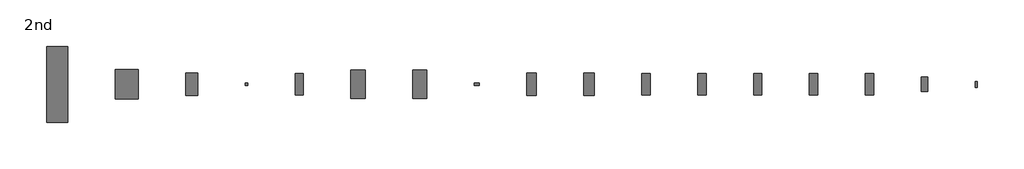
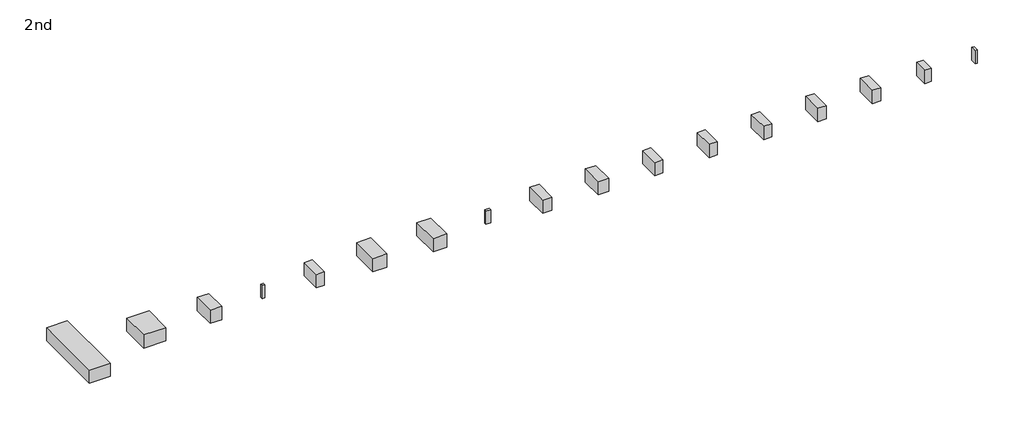
# One storey: 17 proxies.
"""IFC4 building model written with IfcOpenShell, lengths in millimetres."""

import ifcopenshell
import ifcopenshell.guid

model = None  # the IFC model being written
_history = None  # IfcOwnerHistory: only IFC2X3 demands one
_inside = {}  # id of a spatial element -> (the spatial element, [elements in it])
_under = {}  # id of a project, library or spatial element -> (it, [spatial elements below it])
_declared = {}  # id of a project -> (the project, [libraries it declares])
_typed = {}  # id of a type object -> (the type object, [elements of that type])
_made_of = {}  # id of a material, layer set ... -> (it, [elements and type objects made of it])


def new_model(schema):
    """Start an empty IFC model of exactly this schema.

    Asked for "IFC4X3", IfcOpenShell would pick the latest addendum, in which some entities
    have other attributes; the version numbers below select the first issue.
    IFC2X3 requires an IfcOwnerHistory on every rooted entity: one is made here for all.
    """
    global model, _history
    if schema == "IFC4X3":
        model = ifcopenshell.file(schema_version=(4, 3, 0, 0))
    else:
        model = ifcopenshell.file(schema=schema)
    _inside.clear()
    _under.clear()
    _declared.clear()
    _typed.clear()
    _made_of.clear()
    _history = None
    if model.schema == "IFC2X3":
        org = make("IfcOrganization", Name="unknown")
        user = make(
            "IfcPersonAndOrganization",
            ThePerson=make("IfcPerson", FamilyName="unknown"),
            TheOrganization=org,
        )
        app = make(
            "IfcApplication",
            ApplicationDeveloper=org,
            Version="unknown",
            ApplicationFullName="unknown",
            ApplicationIdentifier="unknown",
        )
        _history = make(
            "IfcOwnerHistory",
            OwningUser=user,
            OwningApplication=app,
            ChangeAction="ADDED",
            CreationDate=0,
        )
    return model


def make(cls, **values):
    """One entity of the class cls with the attributes given. An attribute that is None is left unset."""
    return model.create_entity(
        cls, **{name: value for name, value in values.items() if value is not None}
    )


def rooted(cls, **values):
    """An entity with a GlobalId (a new one), such as an element, a storey or a relation."""
    return make(cls, GlobalId=ifcopenshell.guid.new(), OwnerHistory=_history, **values)


def si_unit(unit_type, name, prefix=None):
    """IfcSIUnit, for example si_unit("LENGTHUNIT", "METRE", prefix="MILLI")."""
    return make("IfcSIUnit", UnitType=unit_type, Prefix=prefix, Name=name)


def assignment(units):
    """IfcUnitAssignment: the units of a project."""
    return None if units is None else make("IfcUnitAssignment", Units=units)


def point(xyz):
    """IfcCartesianPoint."""
    return None if xyz is None else make("IfcCartesianPoint", Coordinates=xyz)


def direction(xyz):
    """IfcDirection."""
    return None if xyz is None else make("IfcDirection", DirectionRatios=xyz)


def frame(location, z_axis=None, x_axis=None):
    """IfcAxis2Placement3D, a coordinate frame: its origin and axes. An axis left out is left unset."""
    return make(
        "IfcAxis2Placement3D",
        Location=point(location),
        Axis=direction(z_axis),
        RefDirection=direction(x_axis),
    )


def origin():
    """The frame at (0, 0, 0) with its axes left unset."""
    return frame((0.0, 0.0, 0.0))


def origin_with_axes():
    """The frame at (0, 0, 0) with the z axis (0, 0, 1) and the x axis (1, 0, 0) written out."""
    return frame((0.0, 0.0, 0.0), z_axis=(0.0, 0.0, 1.0), x_axis=(1.0, 0.0, 0.0))


def place(relative_to, where):
    """IfcLocalPlacement: puts the frame where relative to a parent placement (None: the world)."""
    return make(
        "IfcLocalPlacement", PlacementRelTo=relative_to, RelativePlacement=where
    )


def context(
    kind, dimensions, precision=None, world=None, true_north=None, identifier=None
):
    """IfcGeometricRepresentationContext, for example the 3D "Model" context."""
    return make(
        "IfcGeometricRepresentationContext",
        ContextIdentifier=identifier,
        ContextType=kind,
        CoordinateSpaceDimension=dimensions,
        Precision=precision,
        WorldCoordinateSystem=world,
        TrueNorth=true_north,
    )


def project(units=None, contexts=None):
    """IfcProject with its units and contexts."""
    return rooted(
        "IfcProject",
        Name="project",
        RepresentationContexts=contexts,
        UnitsInContext=assignment(units),
    )


def spatial(cls, under=None, at=None, **own):
    """A site, building, storey or space (cls), placed at a placement, below another one or the project."""
    s = rooted(cls, ObjectPlacement=at, **own)
    if under is not None:
        _under.setdefault(under.id(), (under, []))[1].append(s)
    return s


def polyline(points):
    """IfcPolyline through the points."""
    return make("IfcPolyline", Points=[point(p) for p in points])


def outline(outer, holes=None, kind="AREA"):
    """IfcArbitraryClosedProfileDef: a profile drawn as a closed curve; with holes, ...WithVoids."""
    if holes is None:
        return make("IfcArbitraryClosedProfileDef", ProfileType=kind, OuterCurve=outer)
    return make(
        "IfcArbitraryProfileDefWithVoids",
        ProfileType=kind,
        OuterCurve=outer,
        InnerCurves=holes,
    )


def extrude(swept, where, along, depth):
    """IfcExtrudedAreaSolid: the profile swept, set in the frame where, extruded along a direction by depth."""
    return make(
        "IfcExtrudedAreaSolid",
        SweptArea=swept,
        Position=where,
        ExtrudedDirection=direction(along),
        Depth=depth,
    )


def shape(context_of_items, identifier, shape_type, items):
    """IfcShapeRepresentation: the items that make up one representation, for example the "Body"."""
    return make(
        "IfcShapeRepresentation",
        ContextOfItems=context_of_items,
        RepresentationIdentifier=identifier,
        RepresentationType=shape_type,
        Items=items,
    )


def source(mapping_origin, context_of_items, identifier, shape_type, items):
    """IfcRepresentationMap: a shape defined once, which mapped items show again and again."""
    return make(
        "IfcRepresentationMap",
        MappingOrigin=mapping_origin,
        MappedRepresentation=shape(context_of_items, identifier, shape_type, items),
    )


def transform(
    local_origin,
    x_axis=None,
    y_axis=None,
    z_axis=None,
    scale=None,
    scale2=None,
    scale3=None,
    uniform=True,
):
    """IfcCartesianTransformationOperator3D, or its non-uniform kind. x_axis, y_axis, z_axis: its Axis1, 2, 3."""
    if uniform:
        return make(
            "IfcCartesianTransformationOperator3D",
            Axis1=direction(x_axis),
            Axis2=direction(y_axis),
            LocalOrigin=point(local_origin),
            Scale=scale,
            Axis3=direction(z_axis),
        )
    return make(
        "IfcCartesianTransformationOperator3DnonUniform",
        Axis1=direction(x_axis),
        Axis2=direction(y_axis),
        LocalOrigin=point(local_origin),
        Scale=scale,
        Axis3=direction(z_axis),
        Scale2=scale2,
        Scale3=scale3,
    )


def mapped(mapping_source, mapping_target):
    """IfcMappedItem: shows the shape of a source again, moved by a transform."""
    return make(
        "IfcMappedItem", MappingSource=mapping_source, MappingTarget=mapping_target
    )


def made_of(thing, what):
    """Note that an element or type object is made of a material, layer set ...; save() writes the relation."""
    if what is not None:
        _made_of.setdefault(what.id(), (what, []))[1].append(thing)
    return thing


def element(
    cls,
    number,
    at=None,
    inside=None,
    cuts=None,
    type_object=None,
    material=None,
    context=None,
    identifier="Body",
    shape_type=None,
    held_by="IfcProductDefinitionShape",
    body=None,
    shapes=None,
    **own,
):
    """One element of the class cls, such as IfcWall. Its Tag is "e" and its number.

    at: its placement. inside: the storey or other place that contains it. cuts: it is an
    opening in that element (IfcRelVoidsElement). A single representation is given by context,
    identifier, shape_type and body (its items); several are given by shapes. held_by: the class
    of the entity that holds the representations. save() writes the other relations.
    """
    e = rooted(cls, Tag="e%d" % number, ObjectPlacement=at, **own)
    if body is not None:
        shapes = [shape(context, identifier, shape_type, body)]
    if shapes is not None:
        e.Representation = make(held_by, Representations=shapes)
    if inside is not None:
        _inside.setdefault(inside.id(), (inside, []))[1].append(e)
    if cuts is not None:
        rooted(
            "IfcRelVoidsElement", RelatingBuildingElement=cuts, RelatedOpeningElement=e
        )
    if type_object is not None:
        _typed.setdefault(type_object.id(), (type_object, []))[1].append(e)
    return made_of(e, material)


def aggregate(whole, parts):
    """IfcRelAggregates: a whole, such as a stair, and the parts it consists of."""
    return rooted("IfcRelAggregates", RelatingObject=whole, RelatedObjects=parts)


def save(model, path):
    """Write the relations noted so far, then the file.

    IfcRelAggregates (storeys below a building ...), IfcRelContainedInSpatialStructure (elements
    in a storey), IfcRelDefinesByType, IfcRelAssociatesMaterial and IfcRelDeclares: one each for
    every whole, place, type object, material and project.
    """
    for whole, parts in _under.values():
        aggregate(whole, parts)
    for where, things in _inside.values():
        rooted(
            "IfcRelContainedInSpatialStructure",
            RelatedElements=things,
            RelatingStructure=where,
        )
    for kind, things in _typed.values():
        rooted("IfcRelDefinesByType", RelatedObjects=things, RelatingType=kind)
    for what, things in _made_of.values():
        rooted("IfcRelAssociatesMaterial", RelatedObjects=things, RelatingMaterial=what)
    for by, libraries in _declared.values():
        rooted("IfcRelDeclares", RelatingContext=by, RelatedDefinitions=libraries)
    model.write(path)


def space_planning_box_space_planning_box_5634f436(model_context):
    return source(origin(), model_context, "Body", "SweptSolid", [
        extrude(outline(polyline([(1350.0, 3000.0), (1350.0, -3000.0), (-1350.0, -3000.0), (-1350.0, 3000.0), (1350.0, 3000.0)])), origin_with_axes(), (0.0, 0.0, 1.0), 6000.0),
    ])


def space_planning_box_space_planning_box_71e2440f(model_context):
    return source(origin(), model_context, "Body", "SweptSolid", [
        extrude(outline(polyline([(500.0, 1250.0), (500.0, -1250.0), (-500.0, -1250.0), (-500.0, 1250.0), (500.0, 1250.0)])), origin_with_axes(), (0.0, 0.0, 1.0), 6000.0),
    ])


def space_planning_box_space_planning_box_3a820573(model_context):
    return source(origin(), model_context, "Body", "SweptSolid", [
        extrude(outline(polyline([(2000.0, 4750.0), (2000.0, -4750.0), (-2000.0, -4750.0), (-2000.0, 4750.0), (2000.0, 4750.0)])), origin_with_axes(), (0.0, 0.0, 1.0), 6000.0),
    ])


def space_planning_box_space_planning_box_57c7875f(model_context):
    return source(origin(), model_context, "Body", "SweptSolid", [
        extrude(outline(polyline([(4500.0, 16000.0), (4500.0, -16000.0), (-4500.0, -16000.0), (-4500.0, 16000.0), (4500.0, 16000.0)])), origin_with_axes(), (0.0, 0.0, 1.0), 6000.0),
    ])


def space_planning_box_space_planning_box_72d488a7(model_context):
    return source(origin(), model_context, "Body", "SweptSolid", [
        extrude(outline(polyline([(4800.0, 6250.0), (4800.0, -6250.0), (-4800.0, -6250.0), (-4800.0, 6250.0), (4800.0, 6250.0)])), origin_with_axes(), (0.0, 0.0, 1.0), 6000.0),
    ])


def space_planning_box_space_planning_box_7902148a(model_context):
    return source(origin(), model_context, "Body", "SweptSolid", [
        extrude(outline(polyline([(2500.0, 4800.0), (2500.0, -4800.0), (-2500.0, -4800.0), (-2500.0, 4800.0), (2500.0, 4800.0)])), origin_with_axes(), (0.0, 0.0, 1.0), 6000.0),
    ])


def space_planning_box_space_planning_box_ed4b717c(model_context):
    return source(origin(), model_context, "Body", "SweptSolid", [
        extrude(outline(polyline([(500.0, 500.0), (500.0, -500.0), (-500.0, -500.0), (-500.0, 500.0), (500.0, 500.0)])), origin_with_axes(), (0.0, 0.0, 1.0), 6000.0),
    ])


def space_planning_box_space_planning_box_c01b8d6f(model_context):
    return source(origin(), model_context, "Body", "SweptSolid", [
        extrude(outline(polyline([(1750.0, 4500.0), (1750.0, -4500.0), (-1750.0, -4500.0), (-1750.0, 4500.0), (1750.0, 4500.0)])), origin_with_axes(), (0.0, 0.0, 1.0), 6000.0),
    ])


def space_planning_box_space_planning_box_43059f4e(model_context):
    return source(origin(), model_context, "Body", "SweptSolid", [
        extrude(outline(polyline([(3000.0, 6000.0), (3000.0, -6000.0), (-3000.0, -6000.0), (-3000.0, 6000.0), (3000.0, 6000.0)])), origin_with_axes(), (0.0, 0.0, 1.0), 6000.0),
    ])


def space_planning_box_space_planning_box_da00a96f(model_context):
    return source(origin(), model_context, "Body", "SweptSolid", [
        extrude(outline(polyline([(1000.0, 500.0), (1000.0, -500.0), (-1000.0, -500.0), (-1000.0, 500.0), (1000.0, 500.0)])), origin_with_axes(), (0.0, 0.0, 1.0), 6000.0),
    ])


def space_planning_box_space_planning_box_96097b63(model_context):
    return source(origin(), model_context, "Body", "SweptSolid", [
        extrude(outline(polyline([(2250.0, 4800.0), (2250.0, -4800.0), (-2250.0, -4800.0), (-2250.0, 4800.0), (2250.0, 4800.0)])), origin_with_axes(), (0.0, 0.0, 1.0), 6000.0),
    ])


model = new_model("IFC4")

# Units and contexts
model_context = context("Model", 3, world=origin())
ifc_project = project(units=[si_unit("LENGTHUNIT", "METRE", prefix="MILLI")], contexts=[model_context])

# Site, building, storey
site = spatial("IfcSite", under=ifc_project)
building = spatial("IfcBuilding", under=site)
storey = spatial("IfcBuildingStorey", under=building, Name="2nd", Elevation=14000.0)

# Proxies
placement = place(None, origin())
space_planning_box_space_planning_box_shape = space_planning_box_space_planning_box_5634f436(model_context)
element("IfcBuildingElementProxy", 1, Name="Space Planning Box : Space Planning Box", ObjectType="Space Planning Box : Space Planning Box", at=placement, inside=storey, context=model_context, shape_type="MappedRepresentation", body=[
    mapped(space_planning_box_space_planning_box_shape, transform((369450.0, 168000.0, 14000.0), x_axis=(1.0, 0.0, 0.0), y_axis=(0.0, 1.0, 0.0), z_axis=(0.0, 0.0, 1.0))),
])
space_planning_box_space_planning_box_2_shape = space_planning_box_space_planning_box_71e2440f(model_context)
element("IfcBuildingElementProxy", 2, Name="Space Planning Box : Space Planning Box", ObjectType="Space Planning Box : Space Planning Box", at=placement, inside=storey, context=model_context, shape_type="MappedRepresentation", body=[
    mapped(space_planning_box_space_planning_box_2_shape, transform((391300.0, 168000.0, 14000.0), x_axis=(1.0, 0.0, 0.0), y_axis=(0.0, 1.0, 0.0), z_axis=(0.0, 0.0, 1.0))),
])
space_planning_box_space_planning_box_3_shape = space_planning_box_space_planning_box_3a820573(model_context)
element("IfcBuildingElementProxy", 3, Name="Space Planning Box : Space Planning Box", ObjectType="Space Planning Box : Space Planning Box", at=placement, inside=storey, context=model_context, shape_type="MappedRepresentation", body=[
    mapped(space_planning_box_space_planning_box_3_shape, transform((204100.0, 168000.0, 14000.0), x_axis=(1.0, 0.0, 0.0), y_axis=(0.0, 1.0, 0.0), z_axis=(0.0, 0.0, 1.0))),
])
space_planning_box_space_planning_box_4_shape = space_planning_box_space_planning_box_57c7875f(model_context)
element("IfcBuildingElementProxy", 4, Name="Space Planning Box : Space Planning Box", ObjectType="Space Planning Box : Space Planning Box", at=placement, inside=storey, context=model_context, shape_type="MappedRepresentation", body=[
    mapped(space_planning_box_space_planning_box_4_shape, transform((4500.0, 168000.0, 14000.0), x_axis=(1.0, 0.0, 0.0), y_axis=(0.0, 1.0, 0.0), z_axis=(0.0, 0.0, 1.0))),
])
space_planning_box_space_planning_box_5_shape = space_planning_box_space_planning_box_72d488a7(model_context)
element("IfcBuildingElementProxy", 5, Name="Space Planning Box : Space Planning Box", ObjectType="Space Planning Box : Space Planning Box", at=placement, inside=storey, context=model_context, shape_type="MappedRepresentation", body=[
    mapped(space_planning_box_space_planning_box_5_shape, transform((33800.0, 168000.0, 14000.0), x_axis=(1.0, 0.0, 0.0), y_axis=(0.0, 1.0, 0.0), z_axis=(0.0, 0.0, 1.0))),
])
space_planning_box_space_planning_box_6_shape = space_planning_box_space_planning_box_7902148a(model_context)
element("IfcBuildingElementProxy", 6, Name="Space Planning Box : Space Planning Box", ObjectType="Space Planning Box : Space Planning Box", at=placement, inside=storey, context=model_context, shape_type="MappedRepresentation", body=[
    mapped(space_planning_box_space_planning_box_6_shape, transform((61100.0, 168000.0, 14000.0), x_axis=(1.0, 0.0, 0.0), y_axis=(0.0, 1.0, 0.0), z_axis=(0.0, 0.0, 1.0))),
])
space_planning_box_space_planning_box_7_shape = space_planning_box_space_planning_box_ed4b717c(model_context)
element("IfcBuildingElementProxy", 7, Name="Space Planning Box : Space Planning Box", ObjectType="Space Planning Box : Space Planning Box", at=placement, inside=storey, context=model_context, shape_type="MappedRepresentation", body=[
    mapped(space_planning_box_space_planning_box_7_shape, transform((84100.0, 168000.0, 14000.0), x_axis=(1.0, 0.0, 0.0), y_axis=(0.0, 1.0, 0.0), z_axis=(0.0, 0.0, 1.0))),
])
space_planning_box_space_planning_box_8_shape = space_planning_box_space_planning_box_c01b8d6f(model_context)
element("IfcBuildingElementProxy", 8, Name="Space Planning Box : Space Planning Box", ObjectType="Space Planning Box : Space Planning Box", at=placement, inside=storey, context=model_context, shape_type="MappedRepresentation", body=[
    mapped(space_planning_box_space_planning_box_8_shape, transform((106350.0, 168000.0, 14000.0), x_axis=(1.0, 0.0, 0.0), y_axis=(0.0, 1.0, 0.0), z_axis=(0.0, 0.0, 1.0))),
])
element("IfcBuildingElementProxy", 9, Name="Space Planning Box : Space Planning Box", ObjectType="Space Planning Box : Space Planning Box", at=placement, inside=storey, context=model_context, shape_type="MappedRepresentation", body=[
    mapped(space_planning_box_space_planning_box_8_shape, transform((252350.0, 168000.0, 14000.0), x_axis=(1.0, 0.0, 0.0), y_axis=(0.0, 1.0, 0.0), z_axis=(0.0, 0.0, 1.0))),
])
element("IfcBuildingElementProxy", 10, Name="Space Planning Box : Space Planning Box", ObjectType="Space Planning Box : Space Planning Box", at=placement, inside=storey, context=model_context, shape_type="MappedRepresentation", body=[
    mapped(space_planning_box_space_planning_box_8_shape, transform((275850.0, 168000.0, 14000.0), x_axis=(1.0, 0.0, 0.0), y_axis=(0.0, 1.0, 0.0), z_axis=(0.0, 0.0, 1.0))),
])
element("IfcBuildingElementProxy", 11, Name="Space Planning Box : Space Planning Box", ObjectType="Space Planning Box : Space Planning Box", at=placement, inside=storey, context=model_context, shape_type="MappedRepresentation", body=[
    mapped(space_planning_box_space_planning_box_8_shape, transform((299350.0, 168000.0, 14000.0), x_axis=(1.0, 0.0, 0.0), y_axis=(0.0, 1.0, 0.0), z_axis=(0.0, 0.0, 1.0))),
])
element("IfcBuildingElementProxy", 12, Name="Space Planning Box : Space Planning Box", ObjectType="Space Planning Box : Space Planning Box", at=placement, inside=storey, context=model_context, shape_type="MappedRepresentation", body=[
    mapped(space_planning_box_space_planning_box_8_shape, transform((322850.0, 168000.0, 14000.0), x_axis=(1.0, 0.0, 0.0), y_axis=(0.0, 1.0, 0.0), z_axis=(0.0, 0.0, 1.0))),
])
element("IfcBuildingElementProxy", 13, Name="Space Planning Box : Space Planning Box", ObjectType="Space Planning Box : Space Planning Box", at=placement, inside=storey, context=model_context, shape_type="MappedRepresentation", body=[
    mapped(space_planning_box_space_planning_box_8_shape, transform((346350.0, 168000.0, 14000.0), x_axis=(1.0, 0.0, 0.0), y_axis=(0.0, 1.0, 0.0), z_axis=(0.0, 0.0, 1.0))),
])
space_planning_box_space_planning_box_9_shape = space_planning_box_space_planning_box_43059f4e(model_context)
element("IfcBuildingElementProxy", 14, Name="Space Planning Box : Space Planning Box", ObjectType="Space Planning Box : Space Planning Box", at=placement, inside=storey, context=model_context, shape_type="MappedRepresentation", body=[
    mapped(space_planning_box_space_planning_box_9_shape, transform((131100.0, 168000.0, 14000.0), x_axis=(1.0, 0.0, 0.0), y_axis=(0.0, 1.0, 0.0), z_axis=(0.0, 0.0, 1.0))),
])
element("IfcBuildingElementProxy", 15, Name="Space Planning Box : Space Planning Box", ObjectType="Space Planning Box : Space Planning Box", at=placement, inside=storey, context=model_context, shape_type="MappedRepresentation", body=[
    mapped(space_planning_box_space_planning_box_9_shape, transform((157100.0, 168000.0, 14000.0), x_axis=(1.0, 0.0, 0.0), y_axis=(0.0, 1.0, 0.0), z_axis=(0.0, 0.0, 1.0))),
])
space_planning_box_space_planning_box_10_shape = space_planning_box_space_planning_box_da00a96f(model_context)
element("IfcBuildingElementProxy", 16, Name="Space Planning Box : Space Planning Box", ObjectType="Space Planning Box : Space Planning Box", at=placement, inside=storey, context=model_context, shape_type="MappedRepresentation", body=[
    mapped(space_planning_box_space_planning_box_10_shape, transform((181100.0, 168000.0, 14000.0), x_axis=(1.0, 0.0, 0.0), y_axis=(0.0, 1.0, 0.0), z_axis=(0.0, 0.0, 1.0))),
])
space_planning_box_space_planning_box_11_shape = space_planning_box_space_planning_box_96097b63(model_context)
element("IfcBuildingElementProxy", 17, Name="Space Planning Box : Space Planning Box", ObjectType="Space Planning Box : Space Planning Box", at=placement, inside=storey, context=model_context, shape_type="MappedRepresentation", body=[
    mapped(space_planning_box_space_planning_box_11_shape, transform((228350.0, 168000.0, 14000.0), x_axis=(1.0, 0.0, 0.0), y_axis=(0.0, 1.0, 0.0), z_axis=(0.0, 0.0, 1.0))),
])

save(model, "model.ifc")

# Revit data of these elements
# Type "Space Planning Box : Space Planning Box"
#   Type Comments = "..."
#   Room Name [instance default] = "?"
#   Assembly Code = "..."
#   Width [instance default] = 1524 mm
#   Program Area [instance default] = 0 m²
#   Length [instance default] = 1524 mm
#   Height [instance default] = 1524 mm
#   Area [instance default] = 2.32258 m²
#   Fill Color [instance default] = Cyan
#   Default Elevation = 0
# Element 1 (IfcBuildingElementProxy, "Space Planning Box : Space Planning Box")
#   Room Name = "Duct Shaft"
#   Width = 2700 mm
#   Program Area = 16.2 m²
#   Length = 6000 mm
#   Height = 6000 mm
#   Area = 16.2 m²
#   Fill Color = Pink
#   Phase Created = New Construction
#   Materials on its faces: "Pink"
# Element 2 (IfcBuildingElementProxy, "Space Planning Box : Space Planning Box")
#   Room Name = "Pipe Shaft"
#   Width = 1000 mm
#   Program Area = 2.5 m²
#   Length = 2500 mm
#   Height = 6000 mm
#   Area = 2.5 m²
#   Fill Color = Pink
#   Phase Created = New Construction
#   Materials on its faces: "Pink"
# Element 3 (IfcBuildingElementProxy, "Space Planning Box : Space Planning Box")
#   Room Name = "Stairway"
#   Width = 4000 mm
#   Program Area = 38 m²
#   Length = 9500 mm
#   Height = 6000 mm
#   Area = 38 m²
#   Fill Color = Lavender
#   Phase Created = New Construction
#   Materials on its faces: "Lavender"
# Element 4 (IfcBuildingElementProxy, "Space Planning Box : Space Planning Box")
#   Room Name = "Central Control Room"
#   Width = 9000 mm
#   Program Area = 288 m²
#   Length = 32000 mm
#   Height = 6000 mm
#   Area = 288 m²
#   Fill Color = Lime
#   Phase Created = New Construction
#   Materials on its faces: "Lime"
# Element 5 (IfcBuildingElementProxy, "Space Planning Box : Space Planning Box")
#   Room Name = "Engineer Room"
#   Width = 9600 mm
#   Program Area = 120 m²
#   Length = 12500 mm
#   Height = 6000 mm
#   Area = 120 m²
#   Fill Color = Lime
#   Phase Created = New Construction
#   Materials on its faces: "Lime"
# Element 6 (IfcBuildingElementProxy, "Space Planning Box : Space Planning Box")
#   Room Name = "Document Room"
#   Width = 5000 mm
#   Program Area = 48 m²
#   Length = 9600 mm
#   Height = 6000 mm
#   Area = 48 m²
#   Fill Color = Lavender
#   Phase Created = New Construction
#   Materials on its faces: "Lavender"
# Element 7 (IfcBuildingElementProxy, "Space Planning Box : Space Planning Box")
#   Room Name = "Fire Gas Room"
#   Width = 1000 mm
#   Program Area = 0 m²
#   Length = 1000 mm
#   Height = 6000 mm
#   Area = 1 m²
#   Fill Color = Cyan
#   Phase Created = New Construction
#   Materials on its faces: "Cyan"
# Element 8 (IfcBuildingElementProxy, "Space Planning Box : Space Planning Box")
#   Room Name = "Kitch & Lunch Room"
#   Width = 3500 mm
#   Program Area = 31.5 m²
#   Length = 9000 mm
#   Height = 6000 mm
#   Area = 31.5 m²
#   Fill Color = Lavender
#   Phase Created = New Construction
#   Materials on its faces: "Lavender"
# Element 9 (IfcBuildingElementProxy, "Space Planning Box : Space Planning Box")
#   Room Name = "LOTO Office Room"
#   Width = 3500 mm
#   Program Area = 31.5 m²
#   Length = 9000 mm
#   Height = 6000 mm
#   Area = 31.5 m²
#   Fill Color = Lavender
#   Phase Created = New Construction
#   Materials on its faces: "Lavender"
# Element 10 (IfcBuildingElementProxy, "Space Planning Box : Space Planning Box")
#   Room Name = "Shower Room (F)"
#   Width = 3500 mm
#   Program Area = 31.5 m²
#   Length = 9000 mm
#   Height = 6000 mm
#   Area = 31.5 m²
#   Fill Color = Lavender
#   Phase Created = New Construction
#   Materials on its faces: "Lavender"
# Element 11 (IfcBuildingElementProxy, "Space Planning Box : Space Planning Box")
#   Room Name = "Locker Room (F)"
#   Width = 3500 mm
#   Program Area = 31.5 m²
#   Length = 9000 mm
#   Height = 6000 mm
#   Area = 31.5 m²
#   Fill Color = Lavender
#   Phase Created = New Construction
#   Materials on its faces: "Lavender"
# Element 12 (IfcBuildingElementProxy, "Space Planning Box : Space Planning Box")
#   Room Name = "Shower Room (M)"
#   Width = 3500 mm
#   Program Area = 31.5 m²
#   Length = 9000 mm
#   Height = 6000 mm
#   Area = 31.5 m²
#   Fill Color = Lavender
#   Phase Created = New Construction
#   Materials on its faces: "Lavender"
# Element 13 (IfcBuildingElementProxy, "Space Planning Box : Space Planning Box")
#   Room Name = "Locker Room (M)"
#   Width = 3500 mm
#   Program Area = 31.5 m²
#   Length = 9000 mm
#   Height = 6000 mm
#   Area = 31.5 m²
#   Fill Color = Lavender
#   Phase Created = New Construction
#   Materials on its faces: "Lavender"
# Element 14 (IfcBuildingElementProxy, "Space Planning Box : Space Planning Box")
#   Room Name = "Toilet (M)"
#   Width = 6000 mm
#   Program Area = 72 m²
#   Length = 12000 mm
#   Height = 6000 mm
#   Area = 72 m²
#   Fill Color = Lavender
#   Phase Created = New Construction
#   Materials on its faces: "Lavender"
# Element 15 (IfcBuildingElementProxy, "Space Planning Box : Space Planning Box")
#   Room Name = "Toilet (F)"
#   Width = 6000 mm
#   Program Area = 72 m²
#   Length = 12000 mm
#   Height = 6000 mm
#   Area = 72 m²
#   Fill Color = Lavender
#   Phase Created = New Construction
#   Materials on its faces: "Lavender"
# Element 16 (IfcBuildingElementProxy, "Space Planning Box : Space Planning Box")
#   Room Name = "Corridor"
#   Width = 2000 mm
#   Program Area = 0 m²
#   Length = 1000 mm
#   Height = 6000 mm
#   Area = 2 m²
#   Fill Color = Lavender
#   Phase Created = New Construction
#   Materials on its faces: "Lavender"
# Element 17 (IfcBuildingElementProxy, "Space Planning Box : Space Planning Box")
#   Room Name = "Shift Office Room"
#   Width = 4500 mm
#   Program Area = 43.2 m²
#   Length = 9600 mm
#   Height = 6000 mm
#   Area = 43.2 m²
#   Fill Color = Lavender
#   Phase Created = New Construction
#   Materials on its faces: "Lavender"
# Materials
#   "Cyan": class "Generic", colour RGB 0 255 255, transparency 0.2, Cost = 0
#   "Pink": class "Generic", colour RGB 255 105 180, transparency 0.2, Cost = 0
#   "Lavender": class "Generic", colour RGB 186 85 211, transparency 0.2, Cost = 0
#   "Lime": class "Generic", colour RGB 0 255 0, transparency 0.2, Cost = 0
